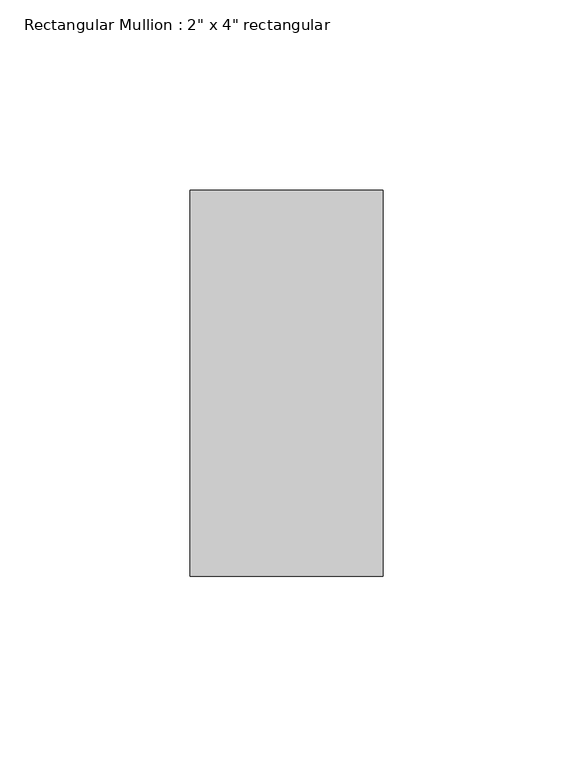
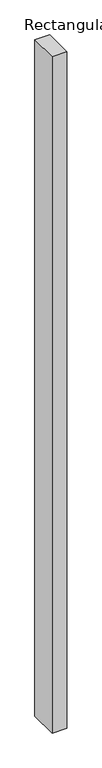
"""IFC4 building model written with IfcOpenShell, lengths in millimetres: member geometry."""

from ifc_helpers import new_model, si_unit, frame, origin, place, context, project, spatial, polyline, outline, extrude, source, transform, mapped, element, save


def member_9a35bcac(model_context):
    return source(origin(), model_context, "Body", "SweptSolid", [
        extrude(outline(polyline([(0.0, 50.8), (0.0, -50.8), (-50.8, -50.8), (-50.8, 50.8), (0.0, 50.8)])), frame((0.0, 0.0, -2438.4), z_axis=(0.0, 0.0, 1.0), x_axis=(1.0, 0.0, 0.0)), (0.0, 0.0, 1.0), 2438.4),
    ])


if __name__ == "__main__":
    model = new_model("IFC4")
    model_context = context("Model", 3, world=origin())
    ifc_project = project(units=[si_unit("LENGTHUNIT", "METRE", prefix="MILLI")], contexts=[model_context])
    site = spatial("IfcSite", under=ifc_project)
    building = spatial("IfcBuilding", under=site)
    placement = place(None, origin())
    member_shape = member_9a35bcac(model_context)
    element("IfcMember", 1, ObjectType="Rectangular Mullion : 2\" x 4\" rectangular", at=placement, inside=building, context=model_context, shape_type="MappedRepresentation", body=[
        mapped(member_shape, transform((0.0, 0.0, 0.0), x_axis=(1.0, 0.0, 0.0), y_axis=(0.0, 1.0, 0.0), z_axis=(0.0, 0.0, 1.0))),
    ])
    save(model, "model.ifc")

# Revit data of these elements
# Type "Rectangular Mullion : 2\" x 4\" rectangular"
#   built-in parameter 1007304 = 0.333333 (stored number, unit not read)
#   built-in parameter 1007301 = 0.0833333 (stored number, unit not read)
#   built-in parameter 1007300 = 0.0833333 (stored number, unit not read)
